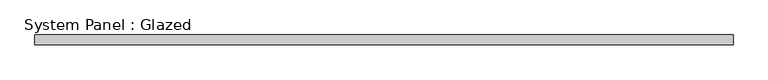
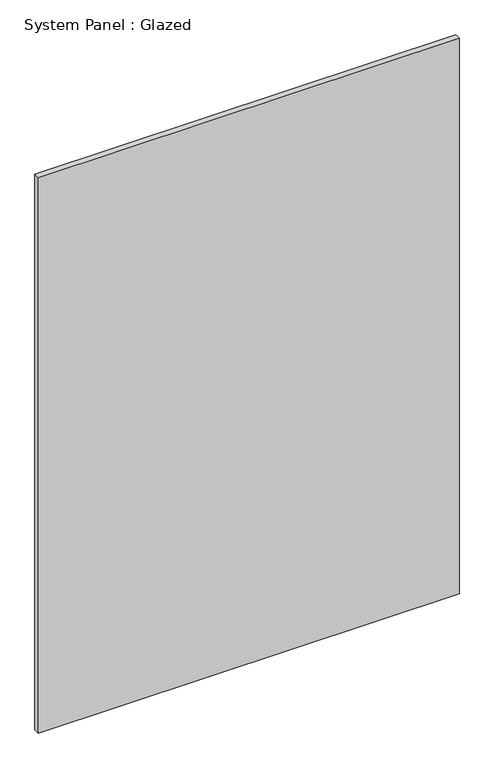
"""IFC4 building model written with IfcOpenShell, lengths in millimetres: plate geometry, System Panel : Glazed."""

from ifc_helpers import new_model, si_unit, origin, origin_with_axes, place, context, project, spatial, polyline, outline, extrude, source, transform, mapped, element, save


def system_panel_glazed_9668c591(model_context):
    return source(origin(), model_context, "Body", "SweptSolid", [
        extrude(outline(polyline([(877.5, 24.5), (-877.5, 24.5), (-877.5, 49.5), (877.5, 49.5), (877.5, 24.5)])), origin_with_axes(), (0.0, 0.0, 1.0), 2450.0),
    ])


if __name__ == "__main__":
    model = new_model("IFC4")
    model_context = context("Model", 3, world=origin())
    ifc_project = project(units=[si_unit("LENGTHUNIT", "METRE", prefix="MILLI")], contexts=[model_context])
    site = spatial("IfcSite", under=ifc_project)
    building = spatial("IfcBuilding", under=site)
    placement = place(None, origin())
    system_panel_glazed_shape = system_panel_glazed_9668c591(model_context)
    element("IfcPlate", 1, ObjectType="System Panel : Glazed", at=placement, inside=building, context=model_context, shape_type="MappedRepresentation", body=[
        mapped(system_panel_glazed_shape, transform((0.0, 0.0, 0.0), x_axis=(1.0, 0.0, 0.0), y_axis=(0.0, 1.0, 0.0), z_axis=(0.0, 0.0, 1.0))),
    ])
    save(model, "model.ifc")

# Revit data of these elements
# Type "System Panel : Glazed"
#   Keynote = "H11"
#   Construction Type Id = "GSP4R"
#   Analytic Construction = "1/8 in Pilkington single glazing"
#   Visual Light Transmittance = 0.9
#   Solar Heat Gain Coefficient = 0.86
#   Heat Transfer Coefficient (U) = 6.7069 W/(m²·K)
# Element 1 (IfcPlate, "System Panel : Glazed")
#   Materials on its faces: "Glass"
# Materials
#   "Glass": class "Glass", colour RGB 0 128 192, transparency 0.9, Description = "Soda Lime Glass", Cost = 0
